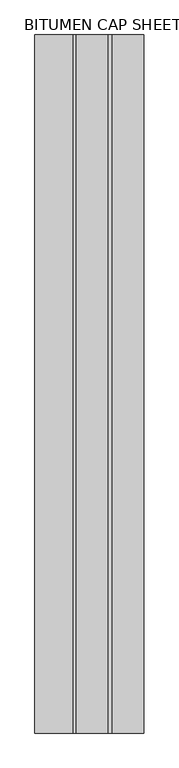
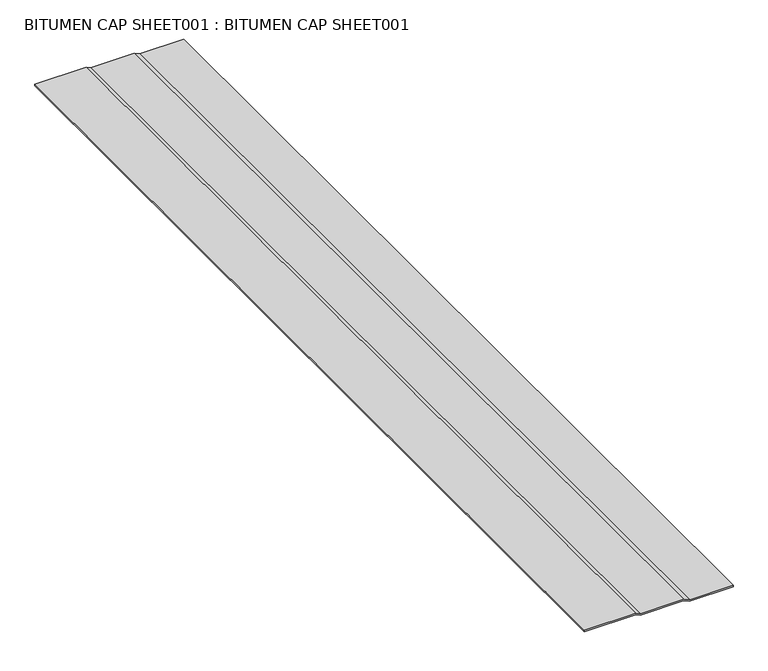
"""IFC4 building model written with IfcOpenShell, lengths in millimetres: proxy geometry, BITUMEN CAP SHEET001 : BITUMEN CAP SHEET001."""

from ifc_helpers import new_model, si_unit, frame, origin, place, context, project, spatial, polyline, outline, extrude, source, transform, mapped, element, save


def bitumen_cap_sheet001_bitumen_cap_sheet001_3f8c56e2(model_context):
    return source(origin(), model_context, "Body", "SweptSolid", [
        extrude(outline(polyline([(40259.2002678, -4699.8063764), (40262.3752678, -4699.8063764), (40262.3752678, -4791.325638), (40267.6612773, -4803.7904566), (40267.6612773, -4894.4742123), (40271.9940719, -4904.1911138), (40271.9940719, -5012.0776104), (40268.8188423, -5012.0776104), (40268.8188423, -4904.8663993), (40264.4862773, -4895.1500128), (40264.4862773, -4804.4358566), (40259.2002678, -4791.971038), (40259.2002678, -4699.8063764)])), frame((0.0, -1052.8906574, 0.0), z_axis=(0.0, 1.0, 0.0), x_axis=(0.0, 0.0, 1.0)), (0.0, 0.0, 1.0), 2000.25),
    ])


if __name__ == "__main__":
    model = new_model("IFC4")
    model_context = context("Model", 3, world=origin())
    ifc_project = project(units=[si_unit("LENGTHUNIT", "METRE", prefix="MILLI")], contexts=[model_context])
    site = spatial("IfcSite", under=ifc_project)
    building = spatial("IfcBuilding", under=site)
    placement = place(None, origin())
    bitumen_cap_sheet001_bitumen_cap_sheet001_shape = bitumen_cap_sheet001_bitumen_cap_sheet001_3f8c56e2(model_context)
    element("IfcBuildingElementProxy", 1, Name="BITUMEN CAP SHEET001 : BITUMEN CAP SHEET001", ObjectType="BITUMEN CAP SHEET001 : BITUMEN CAP SHEET001", at=placement, inside=building, context=model_context, shape_type="MappedRepresentation", body=[
        mapped(bitumen_cap_sheet001_bitumen_cap_sheet001_shape, transform((0.0, 0.0, 0.0), x_axis=(1.0, 0.0, 0.0), y_axis=(0.0, 1.0, 0.0), z_axis=(0.0, 0.0, 1.0))),
    ])
    save(model, "model.ifc")

# Revit data of these elements
# Type "BITUMEN CAP SHEET001 : BITUMEN CAP SHEET001"
#   NameOverride = "BITUMEN CAP SHEET001"
# Element 1 (IfcBuildingElementProxy, "BITUMEN CAP SHEET001 : BITUMEN CAP SHEET001")
#   Materials on its faces: "MODIFIED BITUMEN GRANULE SURFACED CAP SHEET"
# Materials
#   "MODIFIED BITUMEN GRANULE SURFACED CAP SHEET": class "Unassigned", colour RGB 85 85 127, transparency 0
